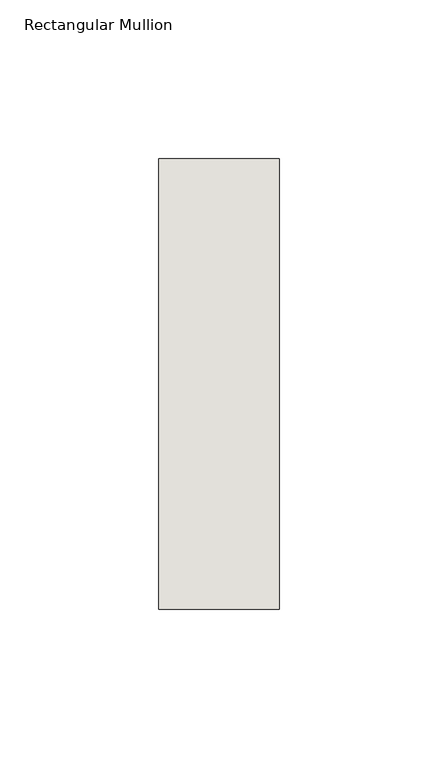
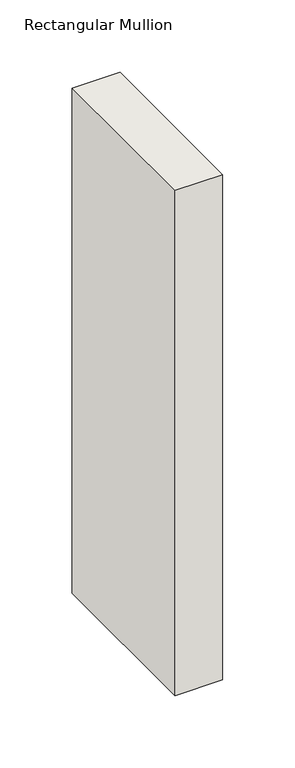
"""IFC4 building model written with IfcOpenShell, lengths in millimetres: wall geometry, Rectangular Mullion : NLRS_21_CWM_hsb-regel 38x142_gen_rsf."""

from ifc_helpers import new_model, si_unit, frame, origin, place, context, project, spatial, polyline, outline, extrude, source, transform, mapped, element, save


def rectangular_mullion_afd5aca7(model_context):
    return source(origin(), model_context, "Body", "SweptSolid", [
        extrude(outline(polyline([(-38.0, -71.0), (-38.0, 71.0), (0.0, 71.0), (0.0, -71.0), (-38.0, -71.0)])), frame((0.0, 0.0, -426.0), z_axis=(0.0, 0.0, 1.0), x_axis=(1.0, 0.0, 0.0)), (0.0, 0.0, 1.0), 426.0),
    ])


if __name__ == "__main__":
    model = new_model("IFC4")
    model_context = context("Model", 3, world=origin())
    ifc_project = project(units=[si_unit("LENGTHUNIT", "METRE", prefix="MILLI")], contexts=[model_context])
    site = spatial("IfcSite", under=ifc_project)
    building = spatial("IfcBuilding", under=site)
    placement = place(None, origin())
    rectangular_mullion_shape = rectangular_mullion_afd5aca7(model_context)
    element("IfcWall", 1, ObjectType="Rectangular Mullion : NLRS_21_CWM_hsb-regel 38x142_gen_rsf", at=placement, inside=building, context=model_context, shape_type="MappedRepresentation", body=[
        mapped(rectangular_mullion_shape, transform((0.0, 0.0, 0.0), x_axis=(1.0, 0.0, 0.0), y_axis=(0.0, 1.0, 0.0), z_axis=(0.0, 0.0, 1.0))),
    ])
    save(model, "model.ifc")

# Revit data of these elements
# Type "Rectangular Mullion : NLRS_21_CWM_hsb-regel 38x142_gen_rsf"
#   Type IfcGUID = "07M7mRoiH1CR8m_RSKIwpF"
#   Assembly Code = "21.10"
#   IfcExportAs = "IfcWall"
#   built-in parameter 1007322 = 0.465879 (stored number, unit not read)
#   built-in parameter 1007321 = 0.062336 (stored number, unit not read)
#   built-in parameter 1007320 = 0.062336 (stored number, unit not read)
# Element 1 (IfcWall, "Rectangular Mullion : NLRS_21_CWM_hsb-regel 38x142_gen_rsf")
#   Materials on its faces: "NLRS_i2_hout naaldhout vuren_gen_rsf"
# Materials
#   "NLRS_i2_hout naaldhout vuren_gen_rsf": class "I - Hout", colour RGB 234 199 147, transparency 0, Keynote = "i2", Manufacturer = "Revit Standards Foundation", URL = "www.revitstandards.org", Description = "hout vuren", Cost = 0
